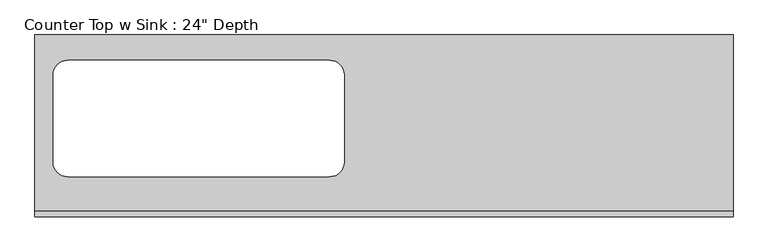
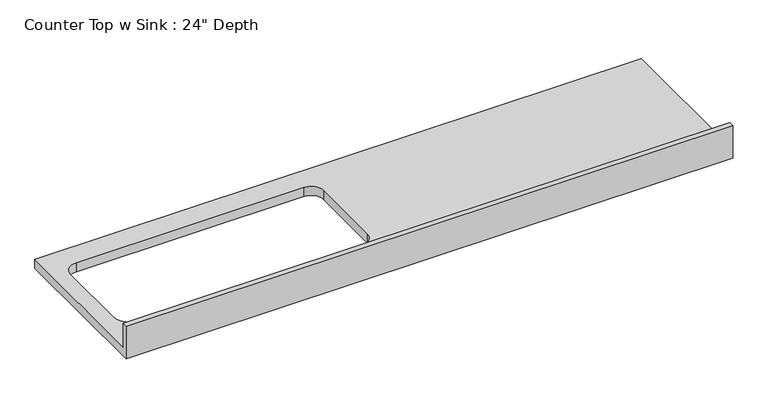
"""IFC4 building model written with IfcOpenShell, lengths in millimetres: furniture geometry."""

import ifcopenshell
import ifcopenshell.guid

model = None  # the IFC model being written
_history = None  # IfcOwnerHistory: only IFC2X3 demands one
_inside = {}  # id of a spatial element -> (the spatial element, [elements in it])
_under = {}  # id of a project, library or spatial element -> (it, [spatial elements below it])
_declared = {}  # id of a project -> (the project, [libraries it declares])
_typed = {}  # id of a type object -> (the type object, [elements of that type])
_made_of = {}  # id of a material, layer set ... -> (it, [elements and type objects made of it])


def new_model(schema):
    """Start an empty IFC model of exactly this schema.

    Asked for "IFC4X3", IfcOpenShell would pick the latest addendum, in which some entities
    have other attributes; the version numbers below select the first issue.
    IFC2X3 requires an IfcOwnerHistory on every rooted entity: one is made here for all.
    """
    global model, _history
    if schema == "IFC4X3":
        model = ifcopenshell.file(schema_version=(4, 3, 0, 0))
    else:
        model = ifcopenshell.file(schema=schema)
    _inside.clear()
    _under.clear()
    _declared.clear()
    _typed.clear()
    _made_of.clear()
    _history = None
    if model.schema == "IFC2X3":
        org = make("IfcOrganization", Name="unknown")
        user = make(
            "IfcPersonAndOrganization",
            ThePerson=make("IfcPerson", FamilyName="unknown"),
            TheOrganization=org,
        )
        app = make(
            "IfcApplication",
            ApplicationDeveloper=org,
            Version="unknown",
            ApplicationFullName="unknown",
            ApplicationIdentifier="unknown",
        )
        _history = make(
            "IfcOwnerHistory",
            OwningUser=user,
            OwningApplication=app,
            ChangeAction="ADDED",
            CreationDate=0,
        )
    return model


def make(cls, **values):
    """One entity of the class cls with the attributes given. An attribute that is None is left unset."""
    return model.create_entity(
        cls, **{name: value for name, value in values.items() if value is not None}
    )


def rooted(cls, **values):
    """An entity with a GlobalId (a new one), such as an element, a storey or a relation."""
    return make(cls, GlobalId=ifcopenshell.guid.new(), OwnerHistory=_history, **values)


def si_unit(unit_type, name, prefix=None):
    """IfcSIUnit, for example si_unit("LENGTHUNIT", "METRE", prefix="MILLI")."""
    return make("IfcSIUnit", UnitType=unit_type, Prefix=prefix, Name=name)


def assignment(units):
    """IfcUnitAssignment: the units of a project."""
    return None if units is None else make("IfcUnitAssignment", Units=units)


def point(xyz):
    """IfcCartesianPoint."""
    return None if xyz is None else make("IfcCartesianPoint", Coordinates=xyz)


def direction(xyz):
    """IfcDirection."""
    return None if xyz is None else make("IfcDirection", DirectionRatios=xyz)


def frame(location, z_axis=None, x_axis=None):
    """IfcAxis2Placement3D, a coordinate frame: its origin and axes. An axis left out is left unset."""
    return make(
        "IfcAxis2Placement3D",
        Location=point(location),
        Axis=direction(z_axis),
        RefDirection=direction(x_axis),
    )


def origin():
    """The frame at (0, 0, 0) with its axes left unset."""
    return frame((0.0, 0.0, 0.0))


def place(relative_to, where):
    """IfcLocalPlacement: puts the frame where relative to a parent placement (None: the world)."""
    return make(
        "IfcLocalPlacement", PlacementRelTo=relative_to, RelativePlacement=where
    )


def context(
    kind, dimensions, precision=None, world=None, true_north=None, identifier=None
):
    """IfcGeometricRepresentationContext, for example the 3D "Model" context."""
    return make(
        "IfcGeometricRepresentationContext",
        ContextIdentifier=identifier,
        ContextType=kind,
        CoordinateSpaceDimension=dimensions,
        Precision=precision,
        WorldCoordinateSystem=world,
        TrueNorth=true_north,
    )


def project(units=None, contexts=None):
    """IfcProject with its units and contexts."""
    return rooted(
        "IfcProject",
        Name="project",
        RepresentationContexts=contexts,
        UnitsInContext=assignment(units),
    )


def spatial(cls, under=None, at=None, **own):
    """A site, building, storey or space (cls), placed at a placement, below another one or the project."""
    s = rooted(cls, ObjectPlacement=at, **own)
    if under is not None:
        _under.setdefault(under.id(), (under, []))[1].append(s)
    return s


def polyline(points):
    """IfcPolyline through the points."""
    return make("IfcPolyline", Points=[point(p) for p in points])


def circle_curve(where, radius):
    """IfcCircle in the frame where."""
    return make("IfcCircle", Position=where, Radius=radius)


def shape(context_of_items, identifier, shape_type, items):
    """IfcShapeRepresentation: the items that make up one representation, for example the "Body"."""
    return make(
        "IfcShapeRepresentation",
        ContextOfItems=context_of_items,
        RepresentationIdentifier=identifier,
        RepresentationType=shape_type,
        Items=items,
    )


def source(mapping_origin, context_of_items, identifier, shape_type, items):
    """IfcRepresentationMap: a shape defined once, which mapped items show again and again."""
    return make(
        "IfcRepresentationMap",
        MappingOrigin=mapping_origin,
        MappedRepresentation=shape(context_of_items, identifier, shape_type, items),
    )


def transform(
    local_origin,
    x_axis=None,
    y_axis=None,
    z_axis=None,
    scale=None,
    scale2=None,
    scale3=None,
    uniform=True,
):
    """IfcCartesianTransformationOperator3D, or its non-uniform kind. x_axis, y_axis, z_axis: its Axis1, 2, 3."""
    if uniform:
        return make(
            "IfcCartesianTransformationOperator3D",
            Axis1=direction(x_axis),
            Axis2=direction(y_axis),
            LocalOrigin=point(local_origin),
            Scale=scale,
            Axis3=direction(z_axis),
        )
    return make(
        "IfcCartesianTransformationOperator3DnonUniform",
        Axis1=direction(x_axis),
        Axis2=direction(y_axis),
        LocalOrigin=point(local_origin),
        Scale=scale,
        Axis3=direction(z_axis),
        Scale2=scale2,
        Scale3=scale3,
    )


def mapped(mapping_source, mapping_target):
    """IfcMappedItem: shows the shape of a source again, moved by a transform."""
    return make(
        "IfcMappedItem", MappingSource=mapping_source, MappingTarget=mapping_target
    )


def made_of(thing, what):
    """Note that an element or type object is made of a material, layer set ...; save() writes the relation."""
    if what is not None:
        _made_of.setdefault(what.id(), (what, []))[1].append(thing)
    return thing


def element(
    cls,
    number,
    at=None,
    inside=None,
    cuts=None,
    type_object=None,
    material=None,
    context=None,
    identifier="Body",
    shape_type=None,
    held_by="IfcProductDefinitionShape",
    body=None,
    shapes=None,
    **own,
):
    """One element of the class cls, such as IfcWall. Its Tag is "e" and its number.

    at: its placement. inside: the storey or other place that contains it. cuts: it is an
    opening in that element (IfcRelVoidsElement). A single representation is given by context,
    identifier, shape_type and body (its items); several are given by shapes. held_by: the class
    of the entity that holds the representations. save() writes the other relations.
    """
    e = rooted(cls, Tag="e%d" % number, ObjectPlacement=at, **own)
    if body is not None:
        shapes = [shape(context, identifier, shape_type, body)]
    if shapes is not None:
        e.Representation = make(held_by, Representations=shapes)
    if inside is not None:
        _inside.setdefault(inside.id(), (inside, []))[1].append(e)
    if cuts is not None:
        rooted(
            "IfcRelVoidsElement", RelatingBuildingElement=cuts, RelatedOpeningElement=e
        )
    if type_object is not None:
        _typed.setdefault(type_object.id(), (type_object, []))[1].append(e)
    return made_of(e, material)


def aggregate(whole, parts):
    """IfcRelAggregates: a whole, such as a stair, and the parts it consists of."""
    return rooted("IfcRelAggregates", RelatingObject=whole, RelatedObjects=parts)


def save(model, path):
    """Write the relations noted so far, then the file.

    IfcRelAggregates (storeys below a building ...), IfcRelContainedInSpatialStructure (elements
    in a storey), IfcRelDefinesByType, IfcRelAssociatesMaterial and IfcRelDeclares: one each for
    every whole, place, type object, material and project.
    """
    for whole, parts in _under.values():
        aggregate(whole, parts)
    for where, things in _inside.values():
        rooted(
            "IfcRelContainedInSpatialStructure",
            RelatedElements=things,
            RelatingStructure=where,
        )
    for kind, things in _typed.values():
        rooted("IfcRelDefinesByType", RelatedObjects=things, RelatingType=kind)
    for what, things in _made_of.values():
        rooted("IfcRelAssociatesMaterial", RelatedObjects=things, RelatingMaterial=what)
    for by, libraries in _declared.values():
        rooted("IfcRelDeclares", RelatingContext=by, RelatedDefinitions=libraries)
    model.write(path)


def plane_surface(at):
    """IfcPlane: the flat surface through the origin of the frame at, square to its z axis."""
    return make("IfcPlane", Position=at)


def revolved_surface(curve, axis_point, axis_direction):
    """IfcSurfaceOfRevolution: the curve turned about the line through axis_point along axis_direction."""
    return make(
        "IfcSurfaceOfRevolution",
        SweptCurve=make("IfcArbitraryOpenProfileDef", ProfileType="CURVE", Curve=curve),
        AxisPosition=make("IfcAxis1Placement", Location=point(axis_point), Axis=direction(axis_direction)),
    )


def advanced_brep(points, edges, surfaces, faces):
    """IfcAdvancedBrep: a solid bounded by faces that lie on surfaces and meet in shared edges.

    An edge is (start, end): straight between two places in points (the first is 0);
    or (start, end, curve); or (start, end, curve, False) where it runs against its curve.
    A face is (place in surfaces, loops), or (place, loops, False) where it looks against
    its surface's normal. A loop lists edges by number (the first is 1), with a minus sign
    where the edge is run from its end to its start. The first loop is the outer one.
    """
    corners = [point(p) for p in points]
    vertices = [make("IfcVertexPoint", VertexGeometry=c) for c in corners]
    made = []
    for start, end, *more in edges:
        made.append(
            make(
                "IfcEdgeCurve",
                EdgeStart=vertices[start],
                EdgeEnd=vertices[end],
                EdgeGeometry=more[0] if more else make("IfcPolyline", Points=[corners[start], corners[end]]),
                SameSense=more[1] if len(more) > 1 else True,
            )
        )
    hull = []
    for where, loops, *sense in faces:
        bounds = []
        for j, loop in enumerate(loops):
            ring = [make("IfcOrientedEdge", EdgeElement=made[abs(k) - 1], Orientation=k > 0) for k in loop]
            bounds.append(
                make(
                    "IfcFaceOuterBound" if j == 0 else "IfcFaceBound",
                    Bound=make("IfcEdgeLoop", EdgeList=ring),
                    Orientation=True,
                )
            )
        hull.append(make("IfcAdvancedFace", Bounds=bounds, FaceSurface=surfaces[where], SameSense=sense[0] if sense else True))
    return make("IfcAdvancedBrep", Outer=make("IfcClosedShell", CfsFaces=hull))


def furniture_ebdcb837(model_context):
    return source(origin(), model_context, "Body", "AdvancedBrep", [
        advanced_brep(
        [(-1200.4622951, 635.0, 914.4), (-1200.4622951, 19.05, 914.4), (1237.9377049, 19.05, 914.4), (1237.9377049, 635.0, 914.4), (-1086.1622951, 139.7, 914.4), (-1136.9622951, 190.5, 914.4), (-1136.9622951, 495.3, 914.4), (-1086.1622951, 546.1, 914.4), (-171.7622951, 546.1, 914.4), (-120.9622951, 495.3, 914.4), (-120.9622951, 190.5, 914.4), (-171.7622951, 139.7, 914.4), (1237.9377049, 0.0, 876.3), (-1200.4622951, 0.0, 876.3), (-1200.4622951, 635.0, 876.3), (1237.9377049, 635.0, 876.3), (-171.7622951, 139.7, 876.3), (-120.9622951, 190.5, 876.3), (-120.9622951, 495.3, 876.3), (-171.7622951, 546.1, 876.3), (-1086.1622951, 546.1, 876.3), (-1136.9622951, 495.3, 876.3), (-1136.9622951, 190.5, 876.3), (-1086.1622951, 139.7, 876.3), (1237.9377049, 0.0, 1016.0), (-1200.4622951, 0.0, 1016.0), (-1200.4622951, 19.05, 1016.0), (1237.9377049, 19.05, 1016.0)],
        [
            (0, 1),
            (1, 2),
            (2, 3),
            (3, 0),
            (4, 5, circle_curve(frame((-1086.1622951, 190.5, 914.4), z_axis=(0.0, 0.0, -1.0), x_axis=(1.0, 0.0, 0.0)), 50.8)),
            (5, 6),
            (6, 7, circle_curve(frame((-1086.1622951, 495.3, 914.4), z_axis=(0.0, 0.0, -1.0), x_axis=(1.0, 0.0, 0.0)), 50.8)),
            (7, 8),
            (8, 9, circle_curve(frame((-171.7622951, 495.3, 914.4), z_axis=(0.0, 0.0, -1.0), x_axis=(1.0, 0.0, 0.0)), 50.8)),
            (9, 10),
            (10, 11, circle_curve(frame((-171.7622951, 190.5, 914.4), z_axis=(0.0, 0.0, -1.0), x_axis=(1.0, 0.0, 0.0)), 50.8)),
            (11, 4),
            (12, 13),
            (13, 14),
            (14, 15),
            (15, 12),
            (16, 17, circle_curve(frame((-171.7622951, 190.5, 876.3), z_axis=(0.0, 0.0, 1.0), x_axis=(1.0, 0.0, 0.0)), 50.8)),
            (17, 18),
            (18, 19, circle_curve(frame((-171.7622951, 495.3, 876.3), z_axis=(0.0, 0.0, 1.0), x_axis=(1.0, 0.0, 0.0)), 50.8)),
            (19, 20),
            (20, 21, circle_curve(frame((-1086.1622951, 495.3, 876.3), z_axis=(0.0, 0.0, 1.0), x_axis=(1.0, 0.0, 0.0)), 50.8)),
            (21, 22),
            (22, 23, circle_curve(frame((-1086.1622951, 190.5, 876.3), z_axis=(0.0, 0.0, 1.0), x_axis=(1.0, 0.0, 0.0)), 50.8)),
            (23, 16),
            (12, 24),
            (24, 25),
            (25, 13),
            (25, 26),
            (26, 1),
            (0, 14),
            (3, 15),
            (2, 27),
            (27, 24),
            (27, 26),
            (11, 16),
            (23, 4),
            (22, 5),
            (21, 6),
            (20, 7),
            (19, 8),
            (18, 9),
            (17, 10),
        ],
        [
            plane_surface(frame((-1200.4622951, 0.0, 914.4), z_axis=(0.0, 0.0, 1.0), x_axis=(-1.0, 0.0, 0.0))),
            plane_surface(frame((-1200.4622951, 0.0, 876.3), z_axis=(0.0, 0.0, -1.0), x_axis=(1.0, 0.0, 0.0))),
            plane_surface(frame((1237.9377049, 0.0, 914.4), z_axis=(0.0, -1.0, 0.0), x_axis=(0.0, 0.0, -1.0))),
            plane_surface(frame((-1200.4622951, 0.0, 914.4), z_axis=(-1.0, 0.0, 0.0), x_axis=(0.0, 0.0, -1.0))),
            plane_surface(frame((-1200.4622951, 635.0, 914.4), z_axis=(0.0, 1.0, 0.0), x_axis=(0.0, 0.0, -1.0))),
            plane_surface(frame((1237.9377049, 635.0, 914.4), z_axis=(1.0, 0.0, 0.0), x_axis=(0.0, 0.0, -1.0))),
            plane_surface(frame((-1200.4622951, 0.0, 1016.0), z_axis=(0.0, 0.0, 1.0), x_axis=(0.0, 1.0, 0.0))),
            plane_surface(frame((-1200.4622951, 19.05, 1016.0), z_axis=(0.0, 1.0, 0.0), x_axis=(0.0, 0.0, -1.0))),
            plane_surface(frame((-171.7622951, 139.7, 914.4), z_axis=(0.0, 1.0, 0.0), x_axis=(0.0, 0.0, -1.0))),
            revolved_surface(polyline([(-1035.3622951, 190.5, 914.4), (-1035.3622951, 190.5, 876.3)]), (-1086.1622951, 190.5, 876.3), (0.0, 0.0, 1.0)),
            plane_surface(frame((-1136.9622951, 190.5, 914.4), z_axis=(1.0, 0.0, 0.0), x_axis=(0.0, 0.0, -1.0))),
            revolved_surface(polyline([(-1035.3622951, 495.3, 914.4), (-1035.3622951, 495.3, 876.3)]), (-1086.1622951, 495.3, 876.3), (0.0, 0.0, 1.0)),
            plane_surface(frame((-1086.1622951, 546.1, 914.4), z_axis=(0.0, -1.0, 0.0), x_axis=(0.0, 0.0, -1.0))),
            revolved_surface(polyline([(-120.96229509999999, 495.3, 914.4), (-120.96229509999999, 495.3, 876.3)]), (-171.7622951, 495.3, 876.3), (0.0, 0.0, 1.0)),
            plane_surface(frame((-120.9622951, 495.3, 914.4), z_axis=(-1.0, 0.0, 0.0), x_axis=(0.0, 0.0, -1.0))),
            revolved_surface(polyline([(-120.96229509999999, 190.5, 914.4), (-120.96229509999999, 190.5, 876.3)]), (-171.7622951, 190.5, 876.3), (0.0, 0.0, 1.0)),
        ],
        [
            (0, [[1, 2, 3, 4], [5, 6, 7, 8, 9, 10, 11, 12]]),
            (1, [[13, 14, 15, 16], [17, 18, 19, 20, 21, 22, 23, 24]]),
            (2, [[25, 26, 27, -13]]),
            (3, [[-27, 28, 29, -1, 30, -14]]),
            (4, [[31, -15, -30, -4]]),
            (5, [[-31, -3, 32, 33, -25, -16]]),
            (6, [[-26, -33, 34, -28]]),
            (7, [[-32, -2, -29, -34]]),
            (8, [[-12, 35, -24, 36]]),
            (9, [[-23, 37, -5, -36]]),
            (10, [[-22, 38, -6, -37]]),
            (11, [[-21, 39, -7, -38]]),
            (12, [[-20, 40, -8, -39]]),
            (13, [[-19, 41, -9, -40]]),
            (14, [[-18, 42, -10, -41]]),
            (15, [[-11, -42, -17, -35]]),
        ],
    ),
    ])


if __name__ == "__main__":
    model = new_model("IFC4")
    model_context = context("Model", 3, world=origin())
    ifc_project = project(units=[si_unit("LENGTHUNIT", "METRE", prefix="MILLI")], contexts=[model_context])
    site = spatial("IfcSite", under=ifc_project)
    building = spatial("IfcBuilding", under=site)
    placement = place(None, origin())
    furniture_shape = furniture_ebdcb837(model_context)
    element("IfcFurniture", 1, ObjectType="Counter Top w Sink : 24\" Depth", at=placement, inside=building, context=model_context, shape_type="MappedRepresentation", body=[
        mapped(furniture_shape, transform((0.0, 0.0, 0.0), x_axis=(1.0, 0.0, 0.0), y_axis=(0.0, 1.0, 0.0), z_axis=(0.0, 0.0, 1.0))),
    ])
    save(model, "model.ifc")

# Revit data of these elements
# Type "Counter Top w Sink : 24\" Depth"
#   Assembly Code = "C1030400"
#   Counter Thickness = 0' - 1 1/2"
#   Depth = 2' - 1"
#   Height = 3' - 0"
#   Length [instance default] = 8' - 0"
#   Sink Location [instance default] = 2' - 0"
#   Sink Location To Wall [instance default] = 0' - 6"
#   Sink Opening Depth [instance default] = 1' - 3"
#   Sink Opening Width [instance default] = 3' - 3"
#   Counter Top Material = none
#   Default Elevation = 0
# Element 1 (IfcFurniture, "Counter Top w Sink : 24\" Depth")
#   Sink Location = 1' - 10 1/2"
#   Materials on its faces: "Laminate"
# Materials
#   "Laminate": class "Unassigned", colour RGB 247 235 201, transparency 0
